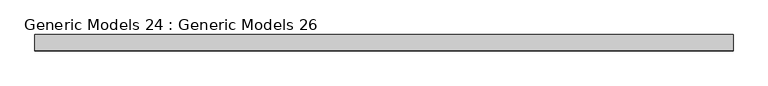
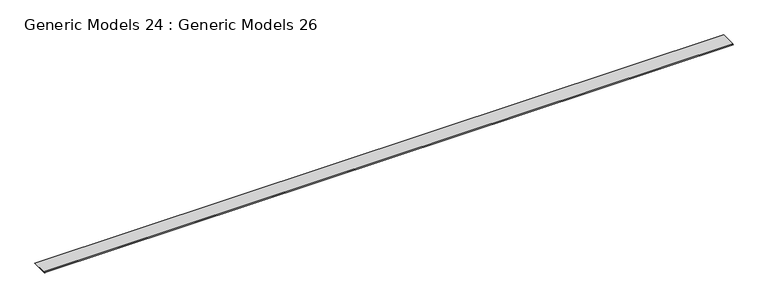
"""IFC4 building model written with IfcOpenShell, lengths in millimetres: proxy geometry, Generic Models 24 : Generic Models 26."""

from ifc_helpers import new_model, si_unit, frame, origin, place, context, project, spatial, polyline, outline, extrude, source, transform, mapped, element, save


def generic_models_24_generic_models_26_a6fb2ab3(model_context):
    return source(origin(), model_context, "Body", "SweptSolid", [
        extrude(outline(polyline([(25633.9840264, 266409.5255146), (25499.0465264, 266409.5255146), (25494.5563983, 266405.0353865), (25493.4338663, 266406.1579186), (25498.3889624, 266411.1130146), (25633.9840264, 266411.1130146), (25633.9840264, 266409.5255146)])), frame((27760.6090778, 0.0, 0.0), z_axis=(1.0, 0.0, 0.0), x_axis=(0.0, 1.0, 0.0)), (0.0, 0.0, 1.0), 6032.7256636),
    ])


if __name__ == "__main__":
    model = new_model("IFC4")
    model_context = context("Model", 3, world=origin())
    ifc_project = project(units=[si_unit("LENGTHUNIT", "METRE", prefix="MILLI")], contexts=[model_context])
    site = spatial("IfcSite", under=ifc_project)
    building = spatial("IfcBuilding", under=site)
    placement = place(None, origin())
    generic_models_24_generic_models_26_shape = generic_models_24_generic_models_26_a6fb2ab3(model_context)
    element("IfcBuildingElementProxy", 1, Name="Generic Models 24 : Generic Models 26", ObjectType="Generic Models 24 : Generic Models 26", at=placement, inside=building, context=model_context, shape_type="MappedRepresentation", body=[
        mapped(generic_models_24_generic_models_26_shape, transform((0.0, 0.0, 0.0), x_axis=(1.0, 0.0, 0.0), y_axis=(0.0, 1.0, 0.0), z_axis=(0.0, 0.0, 1.0))),
    ])
    save(model, "model.ifc")

# Revit data of these elements
# Element 1 (IfcBuildingElementProxy, "Generic Models 24 : Generic Models 26")
#   Materials on its faces: "GALV. BRAKE METAL - (COLOR: DARK BRONZE)"
# Materials
#   "GALV. BRAKE METAL - (COLOR: DARK BRONZE)": class "Generic", colour RGB 72 52 47, transparency 0, Cost = 0
